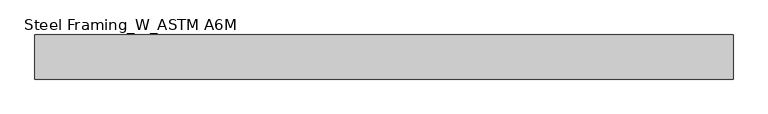
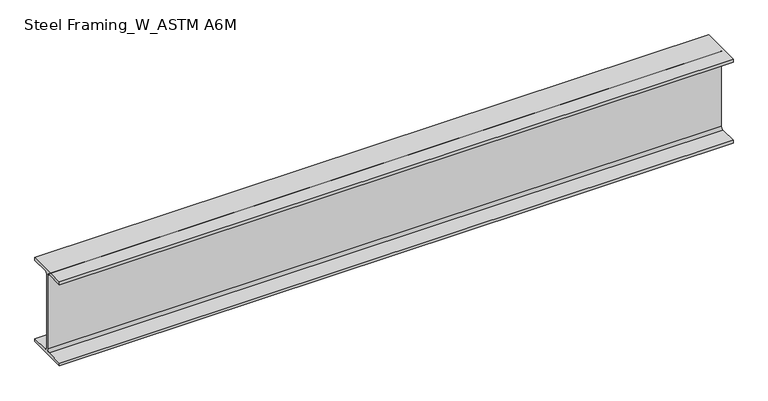
"""IFC4 building model written with IfcOpenShell, lengths in millimetres: beam geometry, Steel Framing_W_ASTM A6M : H_SB_AR_S02_W360x51_G3."""

from ifc_helpers import new_model, si_unit, point, frame, frame_2d, origin, place, context, project, spatial, polyline, circle_curve, trimmed, segment, composite_curve, outline, extrude, source, transform, mapped, element, save


def steel_framing_w_astm_a6m_631b5bf0(model_context):
    return source(origin(), model_context, "Body", "SweptSolid", [
        extrude(outline(composite_curve([segment(polyline([(85.5, -166.4), (85.5, -178.0), (-85.5, -178.0), (-85.5, -166.4), (-13.72, -166.4)]), True, "CONTINUOUS"), segment(trimmed(circle_curve(frame_2d((-13.72, -156.3)), 10.1), [point((-13.72, -166.4))], [point((-3.62, -156.3))], True, "CARTESIAN"), True, "CONTINUOUS"), segment(polyline([(-3.62, -156.3), (-3.62, 156.3)]), True, "CONTINUOUS"), segment(trimmed(circle_curve(frame_2d((-13.72, 156.3)), 10.1), [point((-3.62, 156.3))], [point((-13.72, 166.4))], True, "CARTESIAN"), True, "CONTINUOUS"), segment(polyline([(-13.72, 166.4), (-85.5, 166.4), (-85.5, 178.0), (85.5, 178.0), (85.5, 166.4), (13.72, 166.4)]), True, "CONTINUOUS"), segment(trimmed(circle_curve(frame_2d((13.72, 156.3)), 10.1), [point((13.72, 166.4))], [point((3.62, 156.3))], True, "CARTESIAN"), True, "CONTINUOUS"), segment(polyline([(3.62, 156.3), (3.62, -156.3)]), True, "CONTINUOUS"), segment(trimmed(circle_curve(frame_2d((13.72, -156.3)), 10.1), [point((3.62, -156.3))], [point((13.72, -166.4))], True, "CARTESIAN"), True, "CONTINUOUS"), segment(polyline([(13.72, -166.4), (85.5, -166.4)]), True, "CONTINUOUS")], self_intersect=False)), frame((-1487.2, 0.0, 0.0), z_axis=(1.0, 0.0, 0.0), x_axis=(0.0, 1.0, 0.0)), (0.0, 0.0, 1.0), 2705.1),
    ])


if __name__ == "__main__":
    model = new_model("IFC4")
    model_context = context("Model", 3, world=origin())
    ifc_project = project(units=[si_unit("LENGTHUNIT", "METRE", prefix="MILLI")], contexts=[model_context])
    site = spatial("IfcSite", under=ifc_project)
    building = spatial("IfcBuilding", under=site)
    placement = place(None, origin())
    steel_framing_w_astm_a6m_shape = steel_framing_w_astm_a6m_631b5bf0(model_context)
    element("IfcBeam", 1, ObjectType="Steel Framing_W_ASTM A6M : H_SB_AR_S02_W360x51_G3", at=placement, inside=building, context=model_context, shape_type="MappedRepresentation", body=[
        mapped(steel_framing_w_astm_a6m_shape, transform((0.0, 0.0, 0.0), x_axis=(1.0, 0.0, 0.0), y_axis=(0.0, 1.0, 0.0), z_axis=(0.0, 0.0, 1.0))),
    ])
    save(model, "model.ifc")

# Revit data of these elements
# Type "Steel Framing_W_ASTM A6M : H_SB_AR_S02_W360x51_G3"
#   Type Mark = "G3"
#   Section Name Key = "W14x34"
#   Width = 17.1 cm
#   Web Thickness = 0.724 cm
#   Web Fillet = 1.01 cm
#   Warping Constant = 287000.0 cm⁶
#   Torsional Moment of Inertia = 23.70 cm⁴
#   Section Area = 64.5 cm²
#   Plastic Modulus weak axis = 174.0 cm³
#   Plastic Modulus strong axis = 895.0 cm³
#   Perimeter = 1.36 m²/m
#   Nominal Weight = 51.00 kgf/m
#   Moment of Inertia weak axis = 970.00 cm⁴
#   Moment of Inertia strong axis = 14200.00 cm⁴
#   Height = 35.6 cm
#   Flange Thickness = 1.16 cm
#   Elastic Modulus weak axis = 113.0 cm³
#   Elastic Modulus strong axis = 796.0 cm³
#   Centroid Vertical = 17.8 cm
#   Centroid Horizontal = 8.55 cm
#   Length [instance default] = 1500 mm
#   Structural Material [instance default] = Steel, 45-345
#   Bolt Spacing = 0
#   Assembly Code = ""
# Element 1 (IfcBeam, "Steel Framing_W_ASTM A6M : H_SB_AR_S02_W360x51_G3")
#   Materials on its faces: "Steel, 45-345"
# Materials
#   "Steel, 45-345": class "Metal", colour RGB 189 187 185, transparency 0, Description = "Steel 345 MPa", Cost = 0
